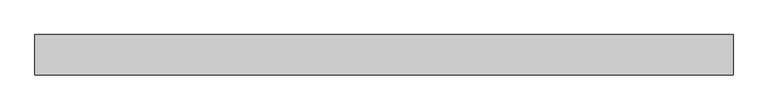
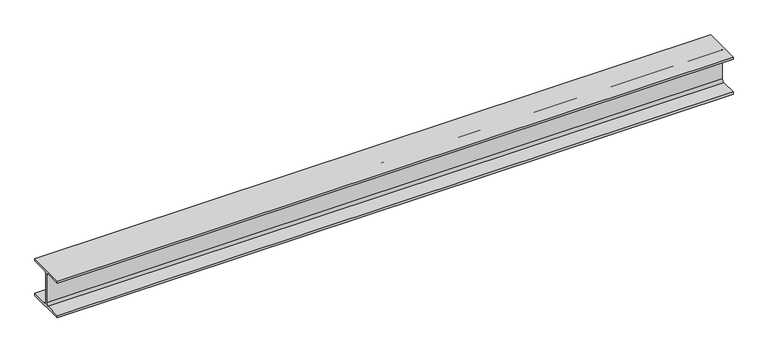
"""IFC4 building model written with IfcOpenShell, lengths in millimetres: beam geometry, 0912_Steel Framing_H-KSD3502 : H_SB_ASB_H-200x200x8x12."""

from ifc_helpers import new_model, si_unit, point, frame, frame_2d, origin, place, context, project, spatial, polyline, circle_curve, trimmed, segment, composite_curve, outline, extrude, source, transform, mapped, element, save


def beam_d92526ff(model_context):
    return source(origin(), model_context, "Body", "SweptSolid", [
        extrude(outline(composite_curve([segment(polyline([(-100.0, -88.0), (-17.0, -88.0)]), True, "CONTINUOUS"), segment(trimmed(circle_curve(frame_2d((-17.0, -75.0)), 13.0), [point((-17.0, -88.0))], [point((-4.0, -75.0))], True, "CARTESIAN"), True, "CONTINUOUS"), segment(polyline([(-4.0, -75.0), (-4.0, 75.0)]), True, "CONTINUOUS"), segment(trimmed(circle_curve(frame_2d((-17.0, 75.0)), 13.0), [point((-4.0, 75.0))], [point((-17.0, 88.0))], True, "CARTESIAN"), True, "CONTINUOUS"), segment(polyline([(-17.0, 88.0), (-100.0, 88.0), (-100.0, 100.0), (100.0, 100.0), (100.0, 88.0), (17.0, 88.0)]), True, "CONTINUOUS"), segment(trimmed(circle_curve(frame_2d((17.0, 75.0)), 13.0), [point((17.0, 88.0))], [point((4.0, 75.0))], True, "CARTESIAN"), True, "CONTINUOUS"), segment(polyline([(4.0, 75.0), (4.0, -75.0)]), True, "CONTINUOUS"), segment(trimmed(circle_curve(frame_2d((17.0, -75.0)), 13.0), [point((4.0, -75.0))], [point((17.0, -88.0))], True, "CARTESIAN"), True, "CONTINUOUS"), segment(polyline([(17.0, -88.0), (100.0, -88.0), (100.0, -100.0), (-100.0, -100.0), (-100.0, -88.0)]), True, "CONTINUOUS")], self_intersect=False)), frame((-1746.373355, 0.0, 0.0), z_axis=(1.0, 0.0, 0.0), x_axis=(0.0, 1.0, 0.0)), (0.0, 0.0, 1.0), 3464.7148219),
    ])


if __name__ == "__main__":
    model = new_model("IFC4")
    model_context = context("Model", 3, world=origin())
    ifc_project = project(units=[si_unit("LENGTHUNIT", "METRE", prefix="MILLI")], contexts=[model_context])
    site = spatial("IfcSite", under=ifc_project)
    building = spatial("IfcBuilding", under=site)
    placement = place(None, origin())
    beam_shape = beam_d92526ff(model_context)
    element("IfcBeam", 1, ObjectType="0912_Steel Framing_H-KSD3502 : H_SB_ASB_H-200x200x8x12", at=placement, inside=building, context=model_context, shape_type="MappedRepresentation", body=[
        mapped(beam_shape, transform((0.0, 0.0, 0.0), x_axis=(1.0, 0.0, 0.0), y_axis=(0.0, 1.0, 0.0), z_axis=(0.0, 0.0, 1.0))),
    ])
    save(model, "model.ifc")

# Revit data of these elements
# Type "0912_Steel Framing_H-KSD3502 : H_SB_ASB_H-200x200x8x12"
#   H_WM Code_1 = "S01AA002-00001 | Main Steel Structure Fabrication Work | Shelter/Building | Medium Steel - Standard (90KG/M>Weight≥30KG/M) | Material: (   )"
#   H_WM Code_2 = "S03AA028-00001 | Main Steel Structure Erection Work | Shelter/Building | Medium Steel (90KG/M>Weight≥30KG/M) | Material: (   )"
#   H_WM Code_3 = "S01AA010-00001 | Main Steel Structure Fabrication Work | Shelter/Building | Steel Painting/Coating | for Non-Fireproofed Steel Surface, Surface Preparation, Primer, Second & Final Coat | Material: (   )"
#   H_Q'ty Cal Type Tag = "SB-Q2"
#   Width = 20.0 cm
#   Web Thickness = 0.8 cm
#   Web Fillet = 1.3 cm
#   Warping Constant = 141000.0 cm⁶
#   W = 0
#   Torsional Moment of Inertia = 26.2485 cm⁴
#   Section Area = 63.53 cm²
#   Plastic Modulus weak axis = 244.0 cm³
#   Plastic Modulus strong axis = 525.0 cm³
#   Perimeter = 1.16 m²/m
#   Nominal Weight = 49.90 kgf/m
#   Moment of Inertia weak axis = 1600.00 cm⁴
#   Moment of Inertia strong axis = 4720.00 cm⁴
#   Height = 20.0 cm
#   Flange Thickness = 1.2 cm
#   Elastic Modulus weak axis = 160.0 cm³
#   Elastic Modulus strong axis = 472.0 cm³
#   Centroid Vertical = 10.0 cm
#   Centroid Horizontal = 10.0 cm
#   Ix = 47200000
#   Length [instance default] = 1.5240 m
#   Zx = 525000
#   b = 0.2000 m
#   h = 0.2000 m
#   r = 0.0130 m
#   s = 0.0080 m
#   t = 0.0120 m
#   A = 0.006353 m²
#   Structural Material [instance default] = Steel, 45-345
#   Assembly Code = ""
# Element 1 (IfcBeam, "0912_Steel Framing_H-KSD3502 : H_SB_ASB_H-200x200x8x12")
#   Structural Material = none
# Materials
#   "Steel, 45-345": class "Metal", colour RGB 189 187 185, transparency 0, Description = "Steel 345 MPa", Cost = 0
